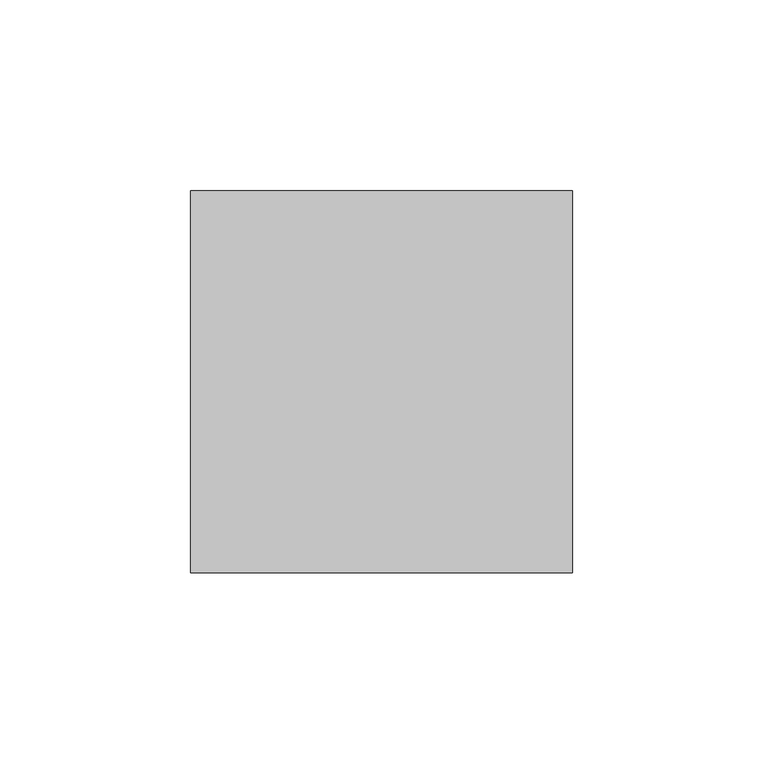
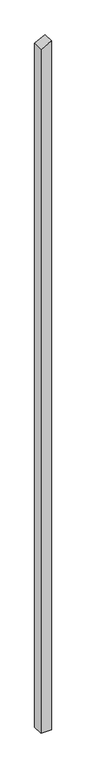
"""IFC4 building model written with IfcOpenShell, lengths in millimetres: column geometry, Holzstütze 159756 : Holzstütze 159756."""

import ifcopenshell
import ifcopenshell.guid

model = None  # the IFC model being written
_history = None  # IfcOwnerHistory: only IFC2X3 demands one
_inside = {}  # id of a spatial element -> (the spatial element, [elements in it])
_under = {}  # id of a project, library or spatial element -> (it, [spatial elements below it])
_declared = {}  # id of a project -> (the project, [libraries it declares])
_typed = {}  # id of a type object -> (the type object, [elements of that type])
_made_of = {}  # id of a material, layer set ... -> (it, [elements and type objects made of it])


def new_model(schema):
    """Start an empty IFC model of exactly this schema.

    Asked for "IFC4X3", IfcOpenShell would pick the latest addendum, in which some entities
    have other attributes; the version numbers below select the first issue.
    IFC2X3 requires an IfcOwnerHistory on every rooted entity: one is made here for all.
    """
    global model, _history
    if schema == "IFC4X3":
        model = ifcopenshell.file(schema_version=(4, 3, 0, 0))
    else:
        model = ifcopenshell.file(schema=schema)
    _inside.clear()
    _under.clear()
    _declared.clear()
    _typed.clear()
    _made_of.clear()
    _history = None
    if model.schema == "IFC2X3":
        org = make("IfcOrganization", Name="unknown")
        user = make(
            "IfcPersonAndOrganization",
            ThePerson=make("IfcPerson", FamilyName="unknown"),
            TheOrganization=org,
        )
        app = make(
            "IfcApplication",
            ApplicationDeveloper=org,
            Version="unknown",
            ApplicationFullName="unknown",
            ApplicationIdentifier="unknown",
        )
        _history = make(
            "IfcOwnerHistory",
            OwningUser=user,
            OwningApplication=app,
            ChangeAction="ADDED",
            CreationDate=0,
        )
    return model


def make(cls, **values):
    """One entity of the class cls with the attributes given. An attribute that is None is left unset."""
    return model.create_entity(
        cls, **{name: value for name, value in values.items() if value is not None}
    )


def rooted(cls, **values):
    """An entity with a GlobalId (a new one), such as an element, a storey or a relation."""
    return make(cls, GlobalId=ifcopenshell.guid.new(), OwnerHistory=_history, **values)


def si_unit(unit_type, name, prefix=None):
    """IfcSIUnit, for example si_unit("LENGTHUNIT", "METRE", prefix="MILLI")."""
    return make("IfcSIUnit", UnitType=unit_type, Prefix=prefix, Name=name)


def assignment(units):
    """IfcUnitAssignment: the units of a project."""
    return None if units is None else make("IfcUnitAssignment", Units=units)


def point(xyz):
    """IfcCartesianPoint."""
    return None if xyz is None else make("IfcCartesianPoint", Coordinates=xyz)


def direction(xyz):
    """IfcDirection."""
    return None if xyz is None else make("IfcDirection", DirectionRatios=xyz)


def frame(location, z_axis=None, x_axis=None):
    """IfcAxis2Placement3D, a coordinate frame: its origin and axes. An axis left out is left unset."""
    return make(
        "IfcAxis2Placement3D",
        Location=point(location),
        Axis=direction(z_axis),
        RefDirection=direction(x_axis),
    )


def origin():
    """The frame at (0, 0, 0) with its axes left unset."""
    return frame((0.0, 0.0, 0.0))


def place(relative_to, where):
    """IfcLocalPlacement: puts the frame where relative to a parent placement (None: the world)."""
    return make(
        "IfcLocalPlacement", PlacementRelTo=relative_to, RelativePlacement=where
    )


def context(
    kind, dimensions, precision=None, world=None, true_north=None, identifier=None
):
    """IfcGeometricRepresentationContext, for example the 3D "Model" context."""
    return make(
        "IfcGeometricRepresentationContext",
        ContextIdentifier=identifier,
        ContextType=kind,
        CoordinateSpaceDimension=dimensions,
        Precision=precision,
        WorldCoordinateSystem=world,
        TrueNorth=true_north,
    )


def project(units=None, contexts=None):
    """IfcProject with its units and contexts."""
    return rooted(
        "IfcProject",
        Name="project",
        RepresentationContexts=contexts,
        UnitsInContext=assignment(units),
    )


def spatial(cls, under=None, at=None, **own):
    """A site, building, storey or space (cls), placed at a placement, below another one or the project."""
    s = rooted(cls, ObjectPlacement=at, **own)
    if under is not None:
        _under.setdefault(under.id(), (under, []))[1].append(s)
    return s


def polyline(points):
    """IfcPolyline through the points."""
    return make("IfcPolyline", Points=[point(p) for p in points])


def outline(outer, holes=None, kind="AREA"):
    """IfcArbitraryClosedProfileDef: a profile drawn as a closed curve; with holes, ...WithVoids."""
    if holes is None:
        return make("IfcArbitraryClosedProfileDef", ProfileType=kind, OuterCurve=outer)
    return make(
        "IfcArbitraryProfileDefWithVoids",
        ProfileType=kind,
        OuterCurve=outer,
        InnerCurves=holes,
    )


def extrude(swept, where, along, depth):
    """IfcExtrudedAreaSolid: the profile swept, set in the frame where, extruded along a direction by depth."""
    return make(
        "IfcExtrudedAreaSolid",
        SweptArea=swept,
        Position=where,
        ExtrudedDirection=direction(along),
        Depth=depth,
    )


def shape(context_of_items, identifier, shape_type, items):
    """IfcShapeRepresentation: the items that make up one representation, for example the "Body"."""
    return make(
        "IfcShapeRepresentation",
        ContextOfItems=context_of_items,
        RepresentationIdentifier=identifier,
        RepresentationType=shape_type,
        Items=items,
    )


def source(mapping_origin, context_of_items, identifier, shape_type, items):
    """IfcRepresentationMap: a shape defined once, which mapped items show again and again."""
    return make(
        "IfcRepresentationMap",
        MappingOrigin=mapping_origin,
        MappedRepresentation=shape(context_of_items, identifier, shape_type, items),
    )


def transform(
    local_origin,
    x_axis=None,
    y_axis=None,
    z_axis=None,
    scale=None,
    scale2=None,
    scale3=None,
    uniform=True,
):
    """IfcCartesianTransformationOperator3D, or its non-uniform kind. x_axis, y_axis, z_axis: its Axis1, 2, 3."""
    if uniform:
        return make(
            "IfcCartesianTransformationOperator3D",
            Axis1=direction(x_axis),
            Axis2=direction(y_axis),
            LocalOrigin=point(local_origin),
            Scale=scale,
            Axis3=direction(z_axis),
        )
    return make(
        "IfcCartesianTransformationOperator3DnonUniform",
        Axis1=direction(x_axis),
        Axis2=direction(y_axis),
        LocalOrigin=point(local_origin),
        Scale=scale,
        Axis3=direction(z_axis),
        Scale2=scale2,
        Scale3=scale3,
    )


def mapped(mapping_source, mapping_target):
    """IfcMappedItem: shows the shape of a source again, moved by a transform."""
    return make(
        "IfcMappedItem", MappingSource=mapping_source, MappingTarget=mapping_target
    )


def made_of(thing, what):
    """Note that an element or type object is made of a material, layer set ...; save() writes the relation."""
    if what is not None:
        _made_of.setdefault(what.id(), (what, []))[1].append(thing)
    return thing


def element(
    cls,
    number,
    at=None,
    inside=None,
    cuts=None,
    type_object=None,
    material=None,
    context=None,
    identifier="Body",
    shape_type=None,
    held_by="IfcProductDefinitionShape",
    body=None,
    shapes=None,
    **own,
):
    """One element of the class cls, such as IfcWall. Its Tag is "e" and its number.

    at: its placement. inside: the storey or other place that contains it. cuts: it is an
    opening in that element (IfcRelVoidsElement). A single representation is given by context,
    identifier, shape_type and body (its items); several are given by shapes. held_by: the class
    of the entity that holds the representations. save() writes the other relations.
    """
    e = rooted(cls, Tag="e%d" % number, ObjectPlacement=at, **own)
    if body is not None:
        shapes = [shape(context, identifier, shape_type, body)]
    if shapes is not None:
        e.Representation = make(held_by, Representations=shapes)
    if inside is not None:
        _inside.setdefault(inside.id(), (inside, []))[1].append(e)
    if cuts is not None:
        rooted(
            "IfcRelVoidsElement", RelatingBuildingElement=cuts, RelatedOpeningElement=e
        )
    if type_object is not None:
        _typed.setdefault(type_object.id(), (type_object, []))[1].append(e)
    return made_of(e, material)


def aggregate(whole, parts):
    """IfcRelAggregates: a whole, such as a stair, and the parts it consists of."""
    return rooted("IfcRelAggregates", RelatingObject=whole, RelatedObjects=parts)


def save(model, path):
    """Write the relations noted so far, then the file.

    IfcRelAggregates (storeys below a building ...), IfcRelContainedInSpatialStructure (elements
    in a storey), IfcRelDefinesByType, IfcRelAssociatesMaterial and IfcRelDeclares: one each for
    every whole, place, type object, material and project.
    """
    for whole, parts in _under.values():
        aggregate(whole, parts)
    for where, things in _inside.values():
        rooted(
            "IfcRelContainedInSpatialStructure",
            RelatedElements=things,
            RelatingStructure=where,
        )
    for kind, things in _typed.values():
        rooted("IfcRelDefinesByType", RelatedObjects=things, RelatingType=kind)
    for what, things in _made_of.values():
        rooted("IfcRelAssociatesMaterial", RelatedObjects=things, RelatingMaterial=what)
    for by, libraries in _declared.values():
        rooted("IfcRelDeclares", RelatingContext=by, RelatedDefinitions=libraries)
    model.write(path)


def column_1855cd1a(model_context):
    return source(origin(), model_context, "Body", "SweptSolid", [
        extrude(outline(polyline([(-500.0, 157297.7593015), (-500.0, 157397.7593015), (6396.6643707, 157397.7593015), (6345.7118258, 157297.7593015), (-500.0, 157297.7593015)])), frame((0.0, 44151.7297978, 0.0), z_axis=(0.0, 1.0, 0.0), x_axis=(0.0, 0.0, 1.0)), (0.0, 0.0, 1.0), 100.0),
    ])


if __name__ == "__main__":
    model = new_model("IFC4")
    model_context = context("Model", 3, world=origin())
    ifc_project = project(units=[si_unit("LENGTHUNIT", "METRE", prefix="MILLI")], contexts=[model_context])
    site = spatial("IfcSite", under=ifc_project)
    building = spatial("IfcBuilding", under=site)
    placement = place(None, origin())
    column_shape = column_1855cd1a(model_context)
    element("IfcColumn", 1, ObjectType="Holzstütze 159756 : Holzstütze 159756", at=placement, inside=building, context=model_context, shape_type="MappedRepresentation", body=[
        mapped(column_shape, transform((0.0, 0.0, 0.0), x_axis=(1.0, 0.0, 0.0), y_axis=(0.0, 1.0, 0.0), z_axis=(0.0, 0.0, 1.0))),
    ])
    save(model, "model.ifc")

# Revit data of these elements
# Type "Holzstütze 159756 : Holzstütze 159756"
#   Abrechnungsart = "m"
#   Allright_Bauteil_ID = "0152St 0000143348"
#   Bezeichnung = "Holzstütze"
#   Codetext = "ST-HOLZ\\"
#   Gewerk = "Zimmer- und Holzbauarbeiten"
#   Material = "Holz"
#   Objektname = "Stütze"
#   NameOverride = "Holzstütze"
#   Reference = "Holzstütze"
#   Status = "NEW"
#   ThermalTransmittance = 0.0000 BTU/(h·ft²·°F)
#   Roll = 0.00°
#   Slope = 0.00°
#   2D Interaktion = yes
#   IsExternal = yes
#   LoadBearing = yes
# Element 1 (IfcColumn, "Holzstütze 159756 : Holzstütze 159756")
#   Materials on its faces: "holzschalung"
# Materials
#   "holzschalung": class "Unassigned", colour RGB 128 128 128, transparency 0
